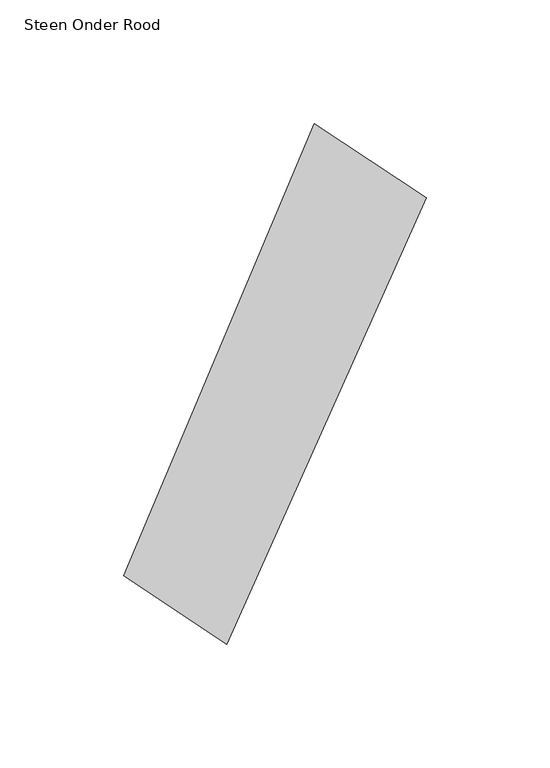
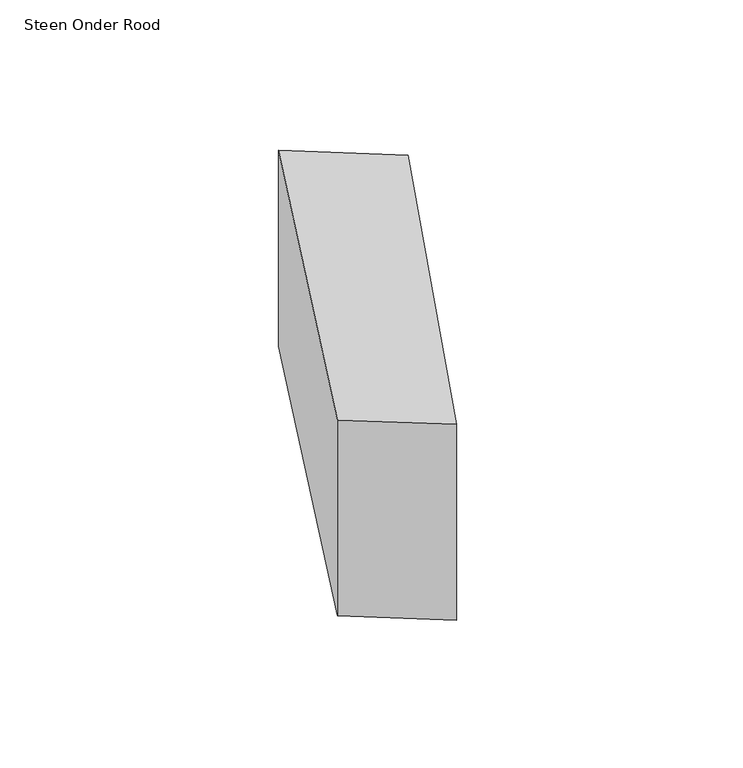
"""IFC4 building model written with IfcOpenShell, lengths in millimetres: proxy geometry, 00_GMA_steen_versie_4 : Steen Onder Rood."""

from ifc_helpers import new_model, si_unit, origin, origin_with_axes, place, context, project, spatial, polyline, outline, extrude, source, transform, mapped, element, save


def steen_onder_rood_ec393941(model_context):
    return source(origin(), model_context, "Body", "SweptSolid", [
        extrude(outline(polyline([(140.726579, 159.3461621), (60.0058242, -21.1898587), (18.3368331, 6.4451766), (95.4508466, 189.3923044), (140.726579, 159.3461621)])), origin_with_axes(), (0.0, 0.0, 1.0), 100.0),
    ])


if __name__ == "__main__":
    model = new_model("IFC4")
    model_context = context("Model", 3, world=origin())
    ifc_project = project(units=[si_unit("LENGTHUNIT", "METRE", prefix="MILLI")], contexts=[model_context])
    site = spatial("IfcSite", under=ifc_project)
    building = spatial("IfcBuilding", under=site)
    placement = place(None, origin())
    steen_onder_rood_shape = steen_onder_rood_ec393941(model_context)
    element("IfcBuildingElementProxy", 1, Name="00_GMA_steen_versie_4 : Steen Onder Rood", ObjectType="00_GMA_steen_versie_4 : Steen Onder Rood", at=placement, inside=building, context=model_context, shape_type="MappedRepresentation", body=[
        mapped(steen_onder_rood_shape, transform((0.0, 0.0, 0.0), x_axis=(1.0, 0.0, 0.0), y_axis=(0.0, 1.0, 0.0), z_axis=(0.0, 0.0, 1.0))),
    ])
    save(model, "model.ifc")

# Revit data of these elements
# Type "00_GMA_steen_versie_4 : Steen Onder Rood"
#   StootVoegHalfBoven [instance default] = 5 mm
#   StootVoegHalf [instance default] = 5 mm
#   StootVoegBreedteOnder = 10 mm
#   StootVoegBreedteBoven = 10 mm
#   Steendikte = 100 mm
#   LintVoegOnderHalf = 0 mm
#   LintVoegOnder = 0 mm
#   LintVoegBovenHalf = 5 mm
#   LintVoegBoven = 10 mm
#   materiaal = 21_steen_rood
#   MateriaalVoeg = none
#   Default Elevation = 0
# Element 1 (IfcBuildingElementProxy, "00_GMA_steen_versie_4 : Steen Onder Rood")
#   Materials on its faces: "21_steen_rood"
# Materials
#   "21_steen_rood": class "Unassigned", colour RGB 213 111 43, transparency 0, Cost = 0
